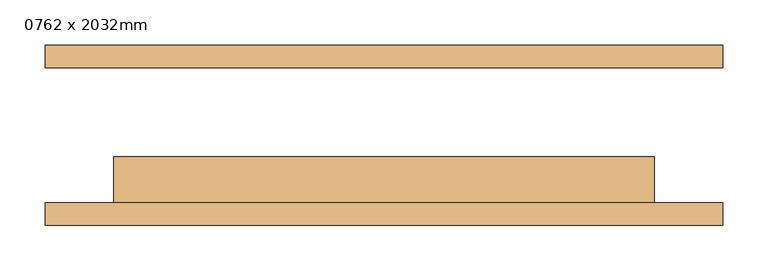
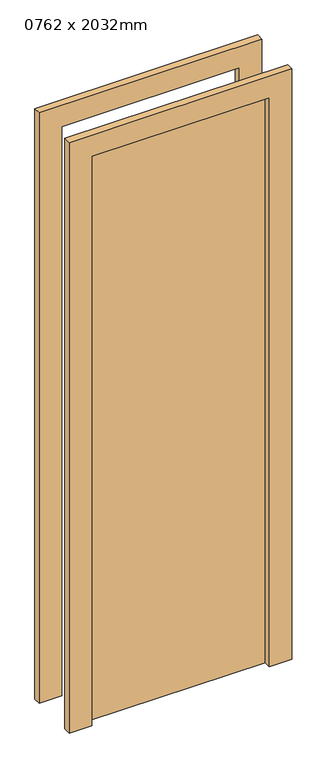
"""IFC4 building model written with IfcOpenShell, lengths in millimetres: door geometry, M_Folha única : 0762 x 2032mm."""

from ifc_helpers import new_model, si_unit, frame, origin, origin_with_axes, place, context, project, spatial, polyline, outline, extrude, source, transform, mapped, element, save


def door_0762_x_2032mm_24b9c1ed(model_context):
    return source(origin(), model_context, "Body", "SweptSolid", [
        extrude(outline(polyline([(2108.0, -376.0), (0.0, -376.0), (0.0, -300.0), (2032.0, -300.0), (2032.0, 300.0), (0.0, 300.0), (0.0, 376.0), (2108.0, 376.0), (2108.0, -376.0)])), frame((0.0, -100.0, 0.0), z_axis=(0.0, 1.0, 0.0), x_axis=(0.0, 0.0, 1.0)), (0.0, 0.0, 1.0), 25.0),
        extrude(outline(polyline([(2108.0, 376.0), (2108.0, -376.0), (0.0, -376.0), (0.0, -300.0), (2032.0, -300.0), (2032.0, 300.0), (0.0, 300.0), (0.0, 376.0), (2108.0, 376.0)])), frame((0.0, 75.0, 0.0), z_axis=(0.0, 1.0, 0.0), x_axis=(0.0, 0.0, 1.0)), (0.0, 0.0, 1.0), 25.0),
        extrude(outline(polyline([(300.0, -24.0), (300.0, -75.0), (-300.0, -75.0), (-300.0, -24.0), (300.0, -24.0)])), origin_with_axes(), (0.0, 0.0, 1.0), 2032.0),
    ])


if __name__ == "__main__":
    model = new_model("IFC4")
    model_context = context("Model", 3, world=origin())
    ifc_project = project(units=[si_unit("LENGTHUNIT", "METRE", prefix="MILLI")], contexts=[model_context])
    site = spatial("IfcSite", under=ifc_project)
    building = spatial("IfcBuilding", under=site)
    placement = place(None, origin())
    door_0762_x_2032mm_shape = door_0762_x_2032mm_24b9c1ed(model_context)
    element("IfcDoor", 1, ObjectType="M_Folha única : 0762 x 2032mm", at=placement, inside=building, context=model_context, shape_type="MappedRepresentation", body=[
        mapped(door_0762_x_2032mm_shape, transform((0.0, 0.0, 0.0), x_axis=(1.0, 0.0, 0.0), y_axis=(0.0, 1.0, 0.0), z_axis=(0.0, 0.0, 1.0))),
    ])
    save(model, "model.ifc")

# Revit data of these elements
# Type "M_Folha única : 0762 x 2032mm"
#   Type Mark = "28"
#   Construction Type Id = "MDOOR"
#   Analytic Construction = "Metal"
#   Thickness = 0.051 m
#   Thermal Resistance (R) = 0.270117 (m²·K)/W
#   Heat Transfer Coefficient (U) = 3.7021 W/(m²·K)
#   Height = 2.032 m
#   Projeção da apara externa = 0.025 m
#   Projeção da apara interna = 0.025 m
#   Largura da apara = 0.076 m
#   Width = 0.60 m
#   Define Thermal Properties by = 1
#   Material da porta = Porta - Painel
#   Material da moldura = Porta - Batente
#   Visual Light Transmittance = 0
#   Solar Heat Gain Coefficient = 0
#   Function = (empty or 0)
#   Wall Closure = (empty or 0)
# Element 1 (IfcDoor, "M_Folha única : 0762 x 2032mm")
#   Materials on its faces: "Porta - Batente", "Porta - Painel"
# Materials
#   "Porta - Painel": class "Madeira", colour RGB 210 159 95, transparency 0, Cost = 0
#   "Porta - Batente": class "Diversos", colour RGB 118 70 51, transparency 0, Cost = 0
